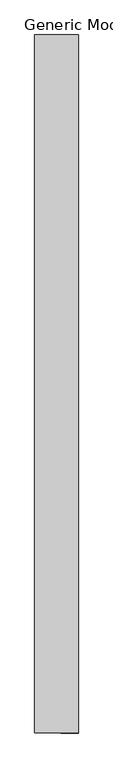
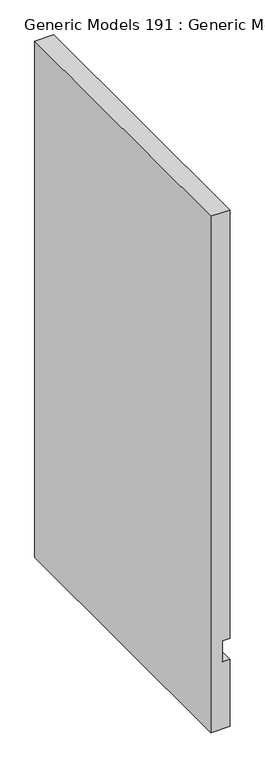
"""IFC4 building model written with IfcOpenShell, lengths in millimetres: proxy geometry, Generic Models 191 : Generic Models 1."""

from ifc_helpers import new_model, si_unit, frame, origin, place, context, project, spatial, polyline, outline, extrude, source, transform, mapped, element, save


def generic_models_191_generic_models_1_83decbcf(model_context):
    return source(origin(), model_context, "Body", "SweptSolid", [
        extrude(outline(polyline([(7.9375, 47261.4625), (7.9375, 47337.6625), (291.1195631, 47337.6625), (291.1195631, 47307.5), (380.0195631, 47307.5), (380.0195631, 47337.6625), (2188.2204978, 47337.6625), (2188.2204978, 47261.4625), (7.9375, 47261.4625)])), frame((0.0, 0.0, 0.0), z_axis=(0.0, 1.0, 0.0), x_axis=(0.0, 0.0, 1.0)), (0.0, 0.0, 1.0), 1219.2),
    ])


if __name__ == "__main__":
    model = new_model("IFC4")
    model_context = context("Model", 3, world=origin())
    ifc_project = project(units=[si_unit("LENGTHUNIT", "METRE", prefix="MILLI")], contexts=[model_context])
    site = spatial("IfcSite", under=ifc_project)
    building = spatial("IfcBuilding", under=site)
    placement = place(None, origin())
    generic_models_191_generic_models_1_shape = generic_models_191_generic_models_1_83decbcf(model_context)
    element("IfcBuildingElementProxy", 1, Name="Generic Models 191 : Generic Models 1", ObjectType="Generic Models 191 : Generic Models 1", at=placement, inside=building, context=model_context, shape_type="MappedRepresentation", body=[
        mapped(generic_models_191_generic_models_1_shape, transform((0.0, 0.0, 0.0), x_axis=(1.0, 0.0, 0.0), y_axis=(0.0, 1.0, 0.0), z_axis=(0.0, 0.0, 1.0))),
    ])
    save(model, "model.ifc")

# Revit data of these elements
# Element 1 (IfcBuildingElementProxy, "Generic Models 191 : Generic Models 1")
#   Materials on its faces: "(S) SOUND BATT. INSULATION (THICKNESS TO MATCH WALL DEPTH)"
# Materials
#   "(S) SOUND BATT. INSULATION (THICKNESS TO MATCH WALL DEPTH)": class "Unassigned", colour RGB 255 255 255, transparency 0, Cost = 0
